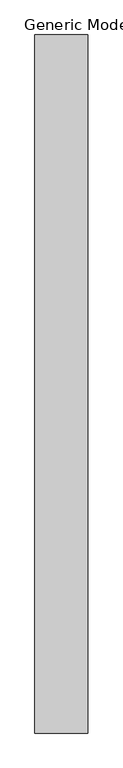
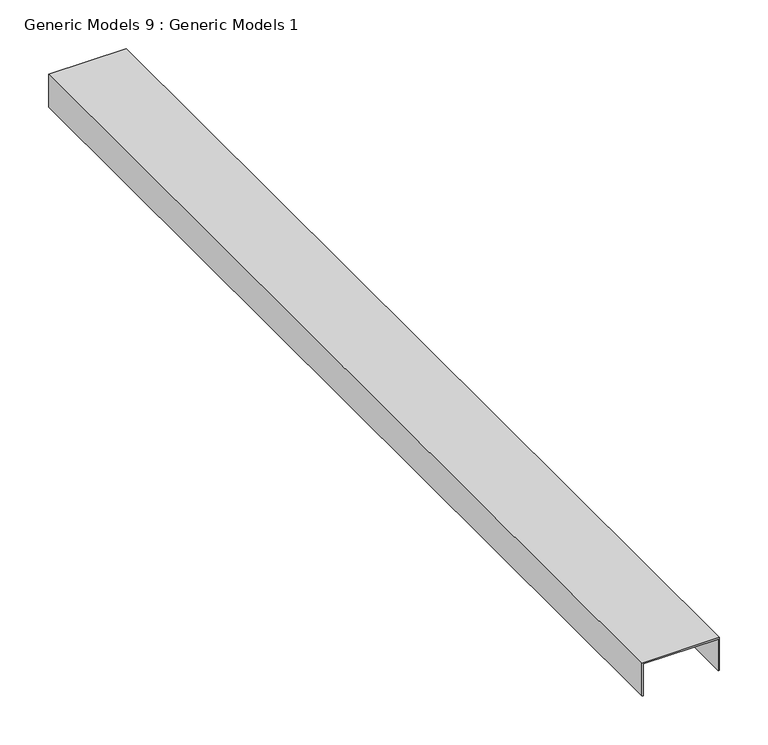
"""IFC4 building model written with IfcOpenShell, lengths in millimetres: proxy geometry, Generic Models 9 : Generic Models 1."""

import ifcopenshell
import ifcopenshell.guid

model = None  # the IFC model being written
_history = None  # IfcOwnerHistory: only IFC2X3 demands one
_inside = {}  # id of a spatial element -> (the spatial element, [elements in it])
_under = {}  # id of a project, library or spatial element -> (it, [spatial elements below it])
_declared = {}  # id of a project -> (the project, [libraries it declares])
_typed = {}  # id of a type object -> (the type object, [elements of that type])
_made_of = {}  # id of a material, layer set ... -> (it, [elements and type objects made of it])


def new_model(schema):
    """Start an empty IFC model of exactly this schema.

    Asked for "IFC4X3", IfcOpenShell would pick the latest addendum, in which some entities
    have other attributes; the version numbers below select the first issue.
    IFC2X3 requires an IfcOwnerHistory on every rooted entity: one is made here for all.
    """
    global model, _history
    if schema == "IFC4X3":
        model = ifcopenshell.file(schema_version=(4, 3, 0, 0))
    else:
        model = ifcopenshell.file(schema=schema)
    _inside.clear()
    _under.clear()
    _declared.clear()
    _typed.clear()
    _made_of.clear()
    _history = None
    if model.schema == "IFC2X3":
        org = make("IfcOrganization", Name="unknown")
        user = make(
            "IfcPersonAndOrganization",
            ThePerson=make("IfcPerson", FamilyName="unknown"),
            TheOrganization=org,
        )
        app = make(
            "IfcApplication",
            ApplicationDeveloper=org,
            Version="unknown",
            ApplicationFullName="unknown",
            ApplicationIdentifier="unknown",
        )
        _history = make(
            "IfcOwnerHistory",
            OwningUser=user,
            OwningApplication=app,
            ChangeAction="ADDED",
            CreationDate=0,
        )
    return model


def make(cls, **values):
    """One entity of the class cls with the attributes given. An attribute that is None is left unset."""
    return model.create_entity(
        cls, **{name: value for name, value in values.items() if value is not None}
    )


def rooted(cls, **values):
    """An entity with a GlobalId (a new one), such as an element, a storey or a relation."""
    return make(cls, GlobalId=ifcopenshell.guid.new(), OwnerHistory=_history, **values)


def si_unit(unit_type, name, prefix=None):
    """IfcSIUnit, for example si_unit("LENGTHUNIT", "METRE", prefix="MILLI")."""
    return make("IfcSIUnit", UnitType=unit_type, Prefix=prefix, Name=name)


def assignment(units):
    """IfcUnitAssignment: the units of a project."""
    return None if units is None else make("IfcUnitAssignment", Units=units)


def point(xyz):
    """IfcCartesianPoint."""
    return None if xyz is None else make("IfcCartesianPoint", Coordinates=xyz)


def direction(xyz):
    """IfcDirection."""
    return None if xyz is None else make("IfcDirection", DirectionRatios=xyz)


def frame(location, z_axis=None, x_axis=None):
    """IfcAxis2Placement3D, a coordinate frame: its origin and axes. An axis left out is left unset."""
    return make(
        "IfcAxis2Placement3D",
        Location=point(location),
        Axis=direction(z_axis),
        RefDirection=direction(x_axis),
    )


def origin():
    """The frame at (0, 0, 0) with its axes left unset."""
    return frame((0.0, 0.0, 0.0))


def place(relative_to, where):
    """IfcLocalPlacement: puts the frame where relative to a parent placement (None: the world)."""
    return make(
        "IfcLocalPlacement", PlacementRelTo=relative_to, RelativePlacement=where
    )


def context(
    kind, dimensions, precision=None, world=None, true_north=None, identifier=None
):
    """IfcGeometricRepresentationContext, for example the 3D "Model" context."""
    return make(
        "IfcGeometricRepresentationContext",
        ContextIdentifier=identifier,
        ContextType=kind,
        CoordinateSpaceDimension=dimensions,
        Precision=precision,
        WorldCoordinateSystem=world,
        TrueNorth=true_north,
    )


def project(units=None, contexts=None):
    """IfcProject with its units and contexts."""
    return rooted(
        "IfcProject",
        Name="project",
        RepresentationContexts=contexts,
        UnitsInContext=assignment(units),
    )


def spatial(cls, under=None, at=None, **own):
    """A site, building, storey or space (cls), placed at a placement, below another one or the project."""
    s = rooted(cls, ObjectPlacement=at, **own)
    if under is not None:
        _under.setdefault(under.id(), (under, []))[1].append(s)
    return s


def polyline(points):
    """IfcPolyline through the points."""
    return make("IfcPolyline", Points=[point(p) for p in points])


def outline(outer, holes=None, kind="AREA"):
    """IfcArbitraryClosedProfileDef: a profile drawn as a closed curve; with holes, ...WithVoids."""
    if holes is None:
        return make("IfcArbitraryClosedProfileDef", ProfileType=kind, OuterCurve=outer)
    return make(
        "IfcArbitraryProfileDefWithVoids",
        ProfileType=kind,
        OuterCurve=outer,
        InnerCurves=holes,
    )


def extrude(swept, where, along, depth):
    """IfcExtrudedAreaSolid: the profile swept, set in the frame where, extruded along a direction by depth."""
    return make(
        "IfcExtrudedAreaSolid",
        SweptArea=swept,
        Position=where,
        ExtrudedDirection=direction(along),
        Depth=depth,
    )


def shape(context_of_items, identifier, shape_type, items):
    """IfcShapeRepresentation: the items that make up one representation, for example the "Body"."""
    return make(
        "IfcShapeRepresentation",
        ContextOfItems=context_of_items,
        RepresentationIdentifier=identifier,
        RepresentationType=shape_type,
        Items=items,
    )


def source(mapping_origin, context_of_items, identifier, shape_type, items):
    """IfcRepresentationMap: a shape defined once, which mapped items show again and again."""
    return make(
        "IfcRepresentationMap",
        MappingOrigin=mapping_origin,
        MappedRepresentation=shape(context_of_items, identifier, shape_type, items),
    )


def transform(
    local_origin,
    x_axis=None,
    y_axis=None,
    z_axis=None,
    scale=None,
    scale2=None,
    scale3=None,
    uniform=True,
):
    """IfcCartesianTransformationOperator3D, or its non-uniform kind. x_axis, y_axis, z_axis: its Axis1, 2, 3."""
    if uniform:
        return make(
            "IfcCartesianTransformationOperator3D",
            Axis1=direction(x_axis),
            Axis2=direction(y_axis),
            LocalOrigin=point(local_origin),
            Scale=scale,
            Axis3=direction(z_axis),
        )
    return make(
        "IfcCartesianTransformationOperator3DnonUniform",
        Axis1=direction(x_axis),
        Axis2=direction(y_axis),
        LocalOrigin=point(local_origin),
        Scale=scale,
        Axis3=direction(z_axis),
        Scale2=scale2,
        Scale3=scale3,
    )


def mapped(mapping_source, mapping_target):
    """IfcMappedItem: shows the shape of a source again, moved by a transform."""
    return make(
        "IfcMappedItem", MappingSource=mapping_source, MappingTarget=mapping_target
    )


def made_of(thing, what):
    """Note that an element or type object is made of a material, layer set ...; save() writes the relation."""
    if what is not None:
        _made_of.setdefault(what.id(), (what, []))[1].append(thing)
    return thing


def element(
    cls,
    number,
    at=None,
    inside=None,
    cuts=None,
    type_object=None,
    material=None,
    context=None,
    identifier="Body",
    shape_type=None,
    held_by="IfcProductDefinitionShape",
    body=None,
    shapes=None,
    **own,
):
    """One element of the class cls, such as IfcWall. Its Tag is "e" and its number.

    at: its placement. inside: the storey or other place that contains it. cuts: it is an
    opening in that element (IfcRelVoidsElement). A single representation is given by context,
    identifier, shape_type and body (its items); several are given by shapes. held_by: the class
    of the entity that holds the representations. save() writes the other relations.
    """
    e = rooted(cls, Tag="e%d" % number, ObjectPlacement=at, **own)
    if body is not None:
        shapes = [shape(context, identifier, shape_type, body)]
    if shapes is not None:
        e.Representation = make(held_by, Representations=shapes)
    if inside is not None:
        _inside.setdefault(inside.id(), (inside, []))[1].append(e)
    if cuts is not None:
        rooted(
            "IfcRelVoidsElement", RelatingBuildingElement=cuts, RelatedOpeningElement=e
        )
    if type_object is not None:
        _typed.setdefault(type_object.id(), (type_object, []))[1].append(e)
    return made_of(e, material)


def aggregate(whole, parts):
    """IfcRelAggregates: a whole, such as a stair, and the parts it consists of."""
    return rooted("IfcRelAggregates", RelatingObject=whole, RelatedObjects=parts)


def save(model, path):
    """Write the relations noted so far, then the file.

    IfcRelAggregates (storeys below a building ...), IfcRelContainedInSpatialStructure (elements
    in a storey), IfcRelDefinesByType, IfcRelAssociatesMaterial and IfcRelDeclares: one each for
    every whole, place, type object, material and project.
    """
    for whole, parts in _under.values():
        aggregate(whole, parts)
    for where, things in _inside.values():
        rooted(
            "IfcRelContainedInSpatialStructure",
            RelatedElements=things,
            RelatingStructure=where,
        )
    for kind, things in _typed.values():
        rooted("IfcRelDefinesByType", RelatedObjects=things, RelatingType=kind)
    for what, things in _made_of.values():
        rooted("IfcRelAssociatesMaterial", RelatedObjects=things, RelatingMaterial=what)
    for by, libraries in _declared.values():
        rooted("IfcRelDeclares", RelatingContext=by, RelatedDefinitions=libraries)
    model.write(path)


def generic_models_9_generic_models_1_a88002d3(model_context):
    return source(origin(), model_context, "Body", "SweptSolid", [
        extrude(outline(polyline([(393.2679367, 51003.2), (393.2679367, 50911.125), (351.9929367, 50911.125), (351.9929367, 50912.7125), (391.6804367, 50912.7125), (391.6804367, 51001.6125), (351.9929367, 51001.6125), (351.9929367, 51003.2), (393.2679367, 51003.2)])), frame((0.0, 0.0, 0.0), z_axis=(0.0, 1.0, 0.0), x_axis=(0.0, 0.0, 1.0)), (0.0, 0.0, 1.0), 1219.2),
    ])


if __name__ == "__main__":
    model = new_model("IFC4")
    model_context = context("Model", 3, world=origin())
    ifc_project = project(units=[si_unit("LENGTHUNIT", "METRE", prefix="MILLI")], contexts=[model_context])
    site = spatial("IfcSite", under=ifc_project)
    building = spatial("IfcBuilding", under=site)
    placement = place(None, origin())
    generic_models_9_generic_models_1_shape = generic_models_9_generic_models_1_a88002d3(model_context)
    element("IfcBuildingElementProxy", 1, Name="Generic Models 9 : Generic Models 1", ObjectType="Generic Models 9 : Generic Models 1", at=placement, inside=building, context=model_context, shape_type="MappedRepresentation", body=[
        mapped(generic_models_9_generic_models_1_shape, transform((0.0, 0.0, 0.0), x_axis=(1.0, 0.0, 0.0), y_axis=(0.0, 1.0, 0.0), z_axis=(0.0, 0.0, 1.0))),
    ])
    save(model, "model.ifc")

# Revit data of these elements
# Element 1 (IfcBuildingElementProxy, "Generic Models 9 : Generic Models 1")
#   Materials on its faces: "METAL RUNNER ANCHORED TO STRUCTURE"
# Materials
#   "METAL RUNNER ANCHORED TO STRUCTURE": class "Unassigned", colour RGB 210 209 208, transparency 0, Keynote = "M05121300.02", Cost = 0
